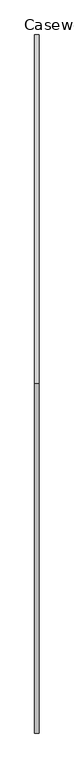
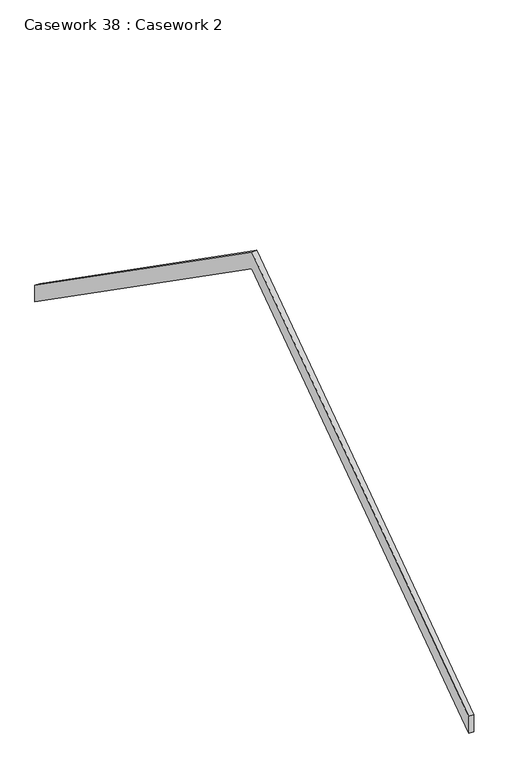
"""IFC4 building model written with IfcOpenShell, lengths in millimetres: furniture geometry, Casework 38 : Casework 2."""

from ifc_helpers import new_model, si_unit, frame, origin, place, context, project, spatial, polyline, outline, extrude, source, transform, mapped, element, save


def casework_38_casework_2_ce946605(model_context):
    return source(origin(), model_context, "Body", "SweptSolid", [
        extrude(outline(polyline([(3152.8649316, 7870.0030963), (7073.1149316, 5125.0144946), (7073.1149316, 4941.8983063), (3152.8649316, 7686.8869079), (-767.3850684, 4941.8983063), (-767.3850684, 5125.0144946), (3152.8649316, 7870.0030963)])), frame((508.4752619, 0.0, 0.0), z_axis=(1.0, 0.0, 0.0), x_axis=(0.0, 1.0, 0.0)), (0.0, 0.0, 1.0), 49.6351915),
    ])


if __name__ == "__main__":
    model = new_model("IFC4")
    model_context = context("Model", 3, world=origin())
    ifc_project = project(units=[si_unit("LENGTHUNIT", "METRE", prefix="MILLI")], contexts=[model_context])
    site = spatial("IfcSite", under=ifc_project)
    building = spatial("IfcBuilding", under=site)
    placement = place(None, origin())
    casework_38_casework_2_shape = casework_38_casework_2_ce946605(model_context)
    element("IfcFurniture", 1, ObjectType="Casework 38 : Casework 2", at=placement, inside=building, context=model_context, shape_type="MappedRepresentation", body=[
        mapped(casework_38_casework_2_shape, transform((0.0, 0.0, 0.0), x_axis=(1.0, 0.0, 0.0), y_axis=(0.0, 1.0, 0.0), z_axis=(0.0, 0.0, 1.0))),
    ])
    save(model, "model.ifc")
